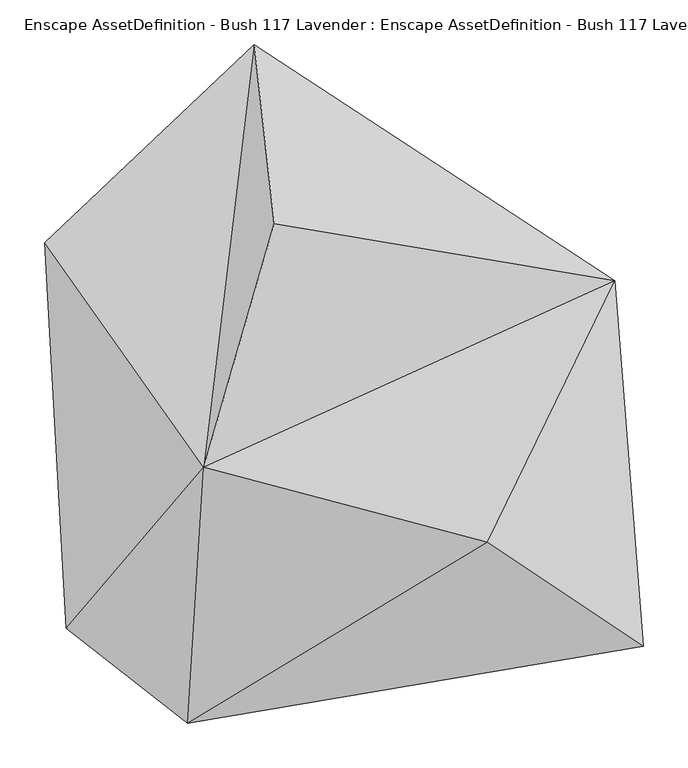
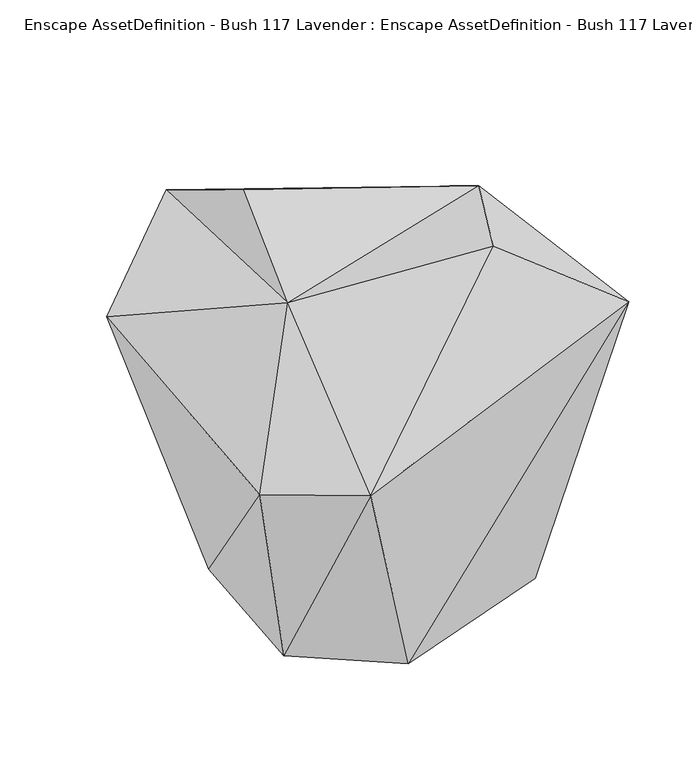
"""IFC4 building model written with IfcOpenShell, lengths in millimetres: geographic element geometry, Enscape AssetDefinition - Bush 117 Lavender : Enscape AssetDefinition - Bush 117 Lavender."""

from ifc_helpers import new_model, si_unit, origin, place, context, project, spatial, faceted_brep, source, transform, mapped, element, save


def enscape_assetdefinition_bush_117_lavender_enscape_4f286e2a(model_context):
    return source(origin(), model_context, "Body", "Brep", [
        faceted_brep([(166.4467156, -115.5674681, 591.4934874), (-169.3107188, -318.253845, 361.6540134), (340.6261802, -232.1405262, 496.9335198), (-151.4145136, -31.9107585, 545.6423163), (-305.3504527, -211.9655013, 346.9774127), (-65.3225183, -254.5777261, -29.0050656), (-221.1816907, -140.365839, -29.0050656), (308.7746799, 176.6777486, 478.8354337), (218.6463922, -154.1026086, -29.0050656), (-72.5895166, 240.4464632, 565.8746958), (-95.0452015, 440.6984746, 452.3712397), (196.9592571, 124.2502853, -29.0050656), (-204.8920393, 119.4176525, -29.0050656), (-67.6226169, 255.9388876, -29.0050656), (-329.3117583, 219.3473428, 429.0544093)], [[[0, 1, 2]], [[3, 1, 0]], [[3, 4, 1]], [[5, 2, 1]], [[6, 1, 4]], [[5, 1, 6]], [[7, 0, 2]], [[8, 2, 5]], [[8, 7, 2]], [[3, 0, 7]], [[7, 9, 3]], [[10, 9, 7]], [[11, 7, 8]], [[11, 10, 7]], [[6, 8, 5]], [[12, 8, 6]], [[13, 8, 12]], [[8, 13, 11]], [[6, 4, 12]], [[12, 14, 13]], [[12, 4, 14]], [[13, 10, 11]], [[13, 14, 10]], [[3, 10, 14]], [[9, 10, 3]], [[3, 14, 4]]]),
    ])


if __name__ == "__main__":
    model = new_model("IFC4")
    model_context = context("Model", 3, world=origin())
    ifc_project = project(units=[si_unit("LENGTHUNIT", "METRE", prefix="MILLI")], contexts=[model_context])
    site = spatial("IfcSite", under=ifc_project)
    building = spatial("IfcBuilding", under=site)
    placement = place(None, origin())
    enscape_assetdefinition_bush_117_lavender_enscape_shape = enscape_assetdefinition_bush_117_lavender_enscape_4f286e2a(model_context)
    element("IfcGeographicElement", 1, ObjectType="Enscape AssetDefinition - Bush 117 Lavender : Enscape AssetDefinition - Bush 117 Lavender", at=placement, inside=building, context=model_context, shape_type="MappedRepresentation", body=[
        mapped(enscape_assetdefinition_bush_117_lavender_enscape_shape, transform((0.0, 0.0, 0.0), x_axis=(1.0, 0.0, 0.0), y_axis=(0.0, 1.0, 0.0), z_axis=(0.0, 0.0, 1.0))),
    ])
    save(model, "model.ifc")

# Revit data of these elements
# Type "Enscape AssetDefinition - Bush 117 Lavender : Enscape AssetDefinition - Bush 117 Lavender"
#   EnscapeAssetSource = "REMOTE"
#   EnscapeAssetId = "13e014c0-ae82-4606-8e21-9cb43f6d8707"
#   Height = 591.493 mm
#   EnscapeNativeAssetHeight = 591.493 mm
#   Default Elevation = 0
